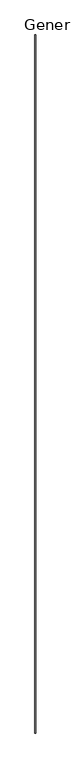
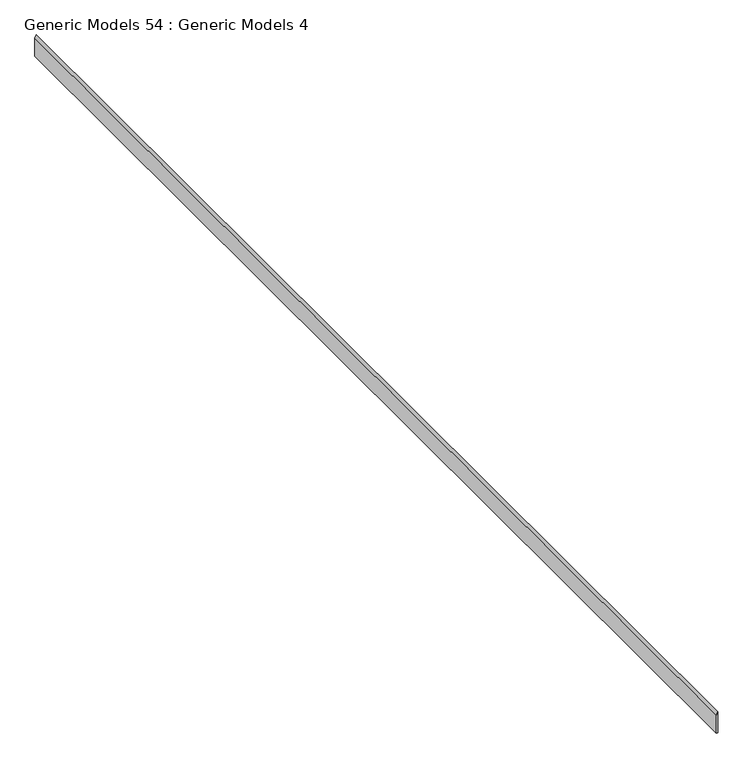
"""IFC4 building model written with IfcOpenShell, lengths in millimetres: proxy geometry, Generic Models 54 : Generic Models 4."""

from ifc_helpers import new_model, si_unit, frame, origin, place, context, project, spatial, polyline, outline, extrude, source, transform, mapped, element, save


def generic_models_54_generic_models_4_bcfbb4ea(model_context):
    return source(origin(), model_context, "Body", "SweptSolid", [
        extrude(outline(polyline([(126914.4742513, -9250.8536295), (126689.866, -9250.8536295), (126689.866, -9234.3436296), (126693.3458, -9234.3436296), (126693.3458, -9233.0736295), (126949.0984618, -9233.0736295), (126914.4742513, -9250.8536295)])), frame((0.0, -6864.9230338, 0.0), z_axis=(0.0, 1.0, 0.0), x_axis=(0.0, 0.0, 1.0)), (0.0, 0.0, 1.0), 13919.2),
    ])


if __name__ == "__main__":
    model = new_model("IFC4")
    model_context = context("Model", 3, world=origin())
    ifc_project = project(units=[si_unit("LENGTHUNIT", "METRE", prefix="MILLI")], contexts=[model_context])
    site = spatial("IfcSite", under=ifc_project)
    building = spatial("IfcBuilding", under=site)
    placement = place(None, origin())
    generic_models_54_generic_models_4_shape = generic_models_54_generic_models_4_bcfbb4ea(model_context)
    element("IfcBuildingElementProxy", 1, Name="Generic Models 54 : Generic Models 4", ObjectType="Generic Models 54 : Generic Models 4", at=placement, inside=building, context=model_context, shape_type="MappedRepresentation", body=[
        mapped(generic_models_54_generic_models_4_shape, transform((0.0, 0.0, 0.0), x_axis=(1.0, 0.0, 0.0), y_axis=(0.0, 1.0, 0.0), z_axis=(0.0, 0.0, 1.0))),
    ])
    save(model, "model.ifc")

# Revit data of these elements
# Element 1 (IfcBuildingElementProxy, "Generic Models 54 : Generic Models 4")
#   Materials on its faces: "_7/8\" SMOOTH TROWEL EXTERIOR STUCCO (COLOR PER OWNER)"
# Materials
#   "_7/8\" SMOOTH TROWEL EXTERIOR STUCCO (COLOR PER OWNER)": class "Generic", colour RGB 233 233 233, transparency 0, Cost = 0
